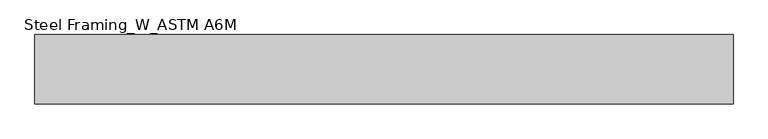
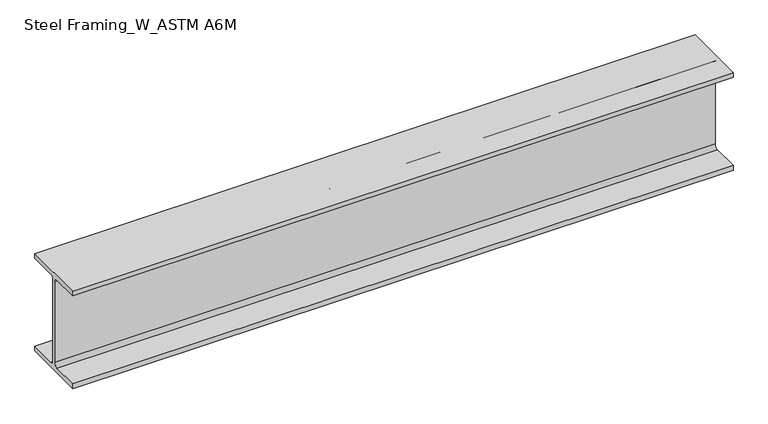
"""IFC4 building model written with IfcOpenShell, lengths in millimetres: beam geometry, Steel Framing_W_ASTM A6M : H_SB_AR_S02_W200x31.3_B6."""

import ifcopenshell
import ifcopenshell.guid

model = None  # the IFC model being written
_history = None  # IfcOwnerHistory: only IFC2X3 demands one
_inside = {}  # id of a spatial element -> (the spatial element, [elements in it])
_under = {}  # id of a project, library or spatial element -> (it, [spatial elements below it])
_declared = {}  # id of a project -> (the project, [libraries it declares])
_typed = {}  # id of a type object -> (the type object, [elements of that type])
_made_of = {}  # id of a material, layer set ... -> (it, [elements and type objects made of it])


def new_model(schema):
    """Start an empty IFC model of exactly this schema.

    Asked for "IFC4X3", IfcOpenShell would pick the latest addendum, in which some entities
    have other attributes; the version numbers below select the first issue.
    IFC2X3 requires an IfcOwnerHistory on every rooted entity: one is made here for all.
    """
    global model, _history
    if schema == "IFC4X3":
        model = ifcopenshell.file(schema_version=(4, 3, 0, 0))
    else:
        model = ifcopenshell.file(schema=schema)
    _inside.clear()
    _under.clear()
    _declared.clear()
    _typed.clear()
    _made_of.clear()
    _history = None
    if model.schema == "IFC2X3":
        org = make("IfcOrganization", Name="unknown")
        user = make(
            "IfcPersonAndOrganization",
            ThePerson=make("IfcPerson", FamilyName="unknown"),
            TheOrganization=org,
        )
        app = make(
            "IfcApplication",
            ApplicationDeveloper=org,
            Version="unknown",
            ApplicationFullName="unknown",
            ApplicationIdentifier="unknown",
        )
        _history = make(
            "IfcOwnerHistory",
            OwningUser=user,
            OwningApplication=app,
            ChangeAction="ADDED",
            CreationDate=0,
        )
    return model


def make(cls, **values):
    """One entity of the class cls with the attributes given. An attribute that is None is left unset."""
    return model.create_entity(
        cls, **{name: value for name, value in values.items() if value is not None}
    )


def rooted(cls, **values):
    """An entity with a GlobalId (a new one), such as an element, a storey or a relation."""
    return make(cls, GlobalId=ifcopenshell.guid.new(), OwnerHistory=_history, **values)


def si_unit(unit_type, name, prefix=None):
    """IfcSIUnit, for example si_unit("LENGTHUNIT", "METRE", prefix="MILLI")."""
    return make("IfcSIUnit", UnitType=unit_type, Prefix=prefix, Name=name)


def assignment(units):
    """IfcUnitAssignment: the units of a project."""
    return None if units is None else make("IfcUnitAssignment", Units=units)


def point(xyz):
    """IfcCartesianPoint."""
    return None if xyz is None else make("IfcCartesianPoint", Coordinates=xyz)


def direction(xyz):
    """IfcDirection."""
    return None if xyz is None else make("IfcDirection", DirectionRatios=xyz)


def frame(location, z_axis=None, x_axis=None):
    """IfcAxis2Placement3D, a coordinate frame: its origin and axes. An axis left out is left unset."""
    return make(
        "IfcAxis2Placement3D",
        Location=point(location),
        Axis=direction(z_axis),
        RefDirection=direction(x_axis),
    )


def frame_2d(location, x_axis=None):
    """IfcAxis2Placement2D, a coordinate frame in the plane: its origin and x axis."""
    return make(
        "IfcAxis2Placement2D", Location=point(location), RefDirection=direction(x_axis)
    )


def origin():
    """The frame at (0, 0, 0) with its axes left unset."""
    return frame((0.0, 0.0, 0.0))


def place(relative_to, where):
    """IfcLocalPlacement: puts the frame where relative to a parent placement (None: the world)."""
    return make(
        "IfcLocalPlacement", PlacementRelTo=relative_to, RelativePlacement=where
    )


def context(
    kind, dimensions, precision=None, world=None, true_north=None, identifier=None
):
    """IfcGeometricRepresentationContext, for example the 3D "Model" context."""
    return make(
        "IfcGeometricRepresentationContext",
        ContextIdentifier=identifier,
        ContextType=kind,
        CoordinateSpaceDimension=dimensions,
        Precision=precision,
        WorldCoordinateSystem=world,
        TrueNorth=true_north,
    )


def project(units=None, contexts=None):
    """IfcProject with its units and contexts."""
    return rooted(
        "IfcProject",
        Name="project",
        RepresentationContexts=contexts,
        UnitsInContext=assignment(units),
    )


def spatial(cls, under=None, at=None, **own):
    """A site, building, storey or space (cls), placed at a placement, below another one or the project."""
    s = rooted(cls, ObjectPlacement=at, **own)
    if under is not None:
        _under.setdefault(under.id(), (under, []))[1].append(s)
    return s


def polyline(points):
    """IfcPolyline through the points."""
    return make("IfcPolyline", Points=[point(p) for p in points])


def circle_curve(where, radius):
    """IfcCircle in the frame where."""
    return make("IfcCircle", Position=where, Radius=radius)


def trimmed(basis, trim1, trim2, sense, master):
    """IfcTrimmedCurve: the piece of a basis curve between two trims."""
    return make(
        "IfcTrimmedCurve",
        BasisCurve=basis,
        Trim1=trim1,
        Trim2=trim2,
        SenseAgreement=sense,
        MasterRepresentation=master,
    )


def segment(curve, same_sense, transition):
    """IfcCompositeCurveSegment."""
    return make(
        "IfcCompositeCurveSegment",
        Transition=transition,
        SameSense=same_sense,
        ParentCurve=curve,
    )


def composite_curve(segments, self_intersect=None):
    """IfcCompositeCurve: segments joined end to end."""
    return make("IfcCompositeCurve", Segments=segments, SelfIntersect=self_intersect)


def outline(outer, holes=None, kind="AREA"):
    """IfcArbitraryClosedProfileDef: a profile drawn as a closed curve; with holes, ...WithVoids."""
    if holes is None:
        return make("IfcArbitraryClosedProfileDef", ProfileType=kind, OuterCurve=outer)
    return make(
        "IfcArbitraryProfileDefWithVoids",
        ProfileType=kind,
        OuterCurve=outer,
        InnerCurves=holes,
    )


def extrude(swept, where, along, depth):
    """IfcExtrudedAreaSolid: the profile swept, set in the frame where, extruded along a direction by depth."""
    return make(
        "IfcExtrudedAreaSolid",
        SweptArea=swept,
        Position=where,
        ExtrudedDirection=direction(along),
        Depth=depth,
    )


def shape(context_of_items, identifier, shape_type, items):
    """IfcShapeRepresentation: the items that make up one representation, for example the "Body"."""
    return make(
        "IfcShapeRepresentation",
        ContextOfItems=context_of_items,
        RepresentationIdentifier=identifier,
        RepresentationType=shape_type,
        Items=items,
    )


def source(mapping_origin, context_of_items, identifier, shape_type, items):
    """IfcRepresentationMap: a shape defined once, which mapped items show again and again."""
    return make(
        "IfcRepresentationMap",
        MappingOrigin=mapping_origin,
        MappedRepresentation=shape(context_of_items, identifier, shape_type, items),
    )


def transform(
    local_origin,
    x_axis=None,
    y_axis=None,
    z_axis=None,
    scale=None,
    scale2=None,
    scale3=None,
    uniform=True,
):
    """IfcCartesianTransformationOperator3D, or its non-uniform kind. x_axis, y_axis, z_axis: its Axis1, 2, 3."""
    if uniform:
        return make(
            "IfcCartesianTransformationOperator3D",
            Axis1=direction(x_axis),
            Axis2=direction(y_axis),
            LocalOrigin=point(local_origin),
            Scale=scale,
            Axis3=direction(z_axis),
        )
    return make(
        "IfcCartesianTransformationOperator3DnonUniform",
        Axis1=direction(x_axis),
        Axis2=direction(y_axis),
        LocalOrigin=point(local_origin),
        Scale=scale,
        Axis3=direction(z_axis),
        Scale2=scale2,
        Scale3=scale3,
    )


def mapped(mapping_source, mapping_target):
    """IfcMappedItem: shows the shape of a source again, moved by a transform."""
    return make(
        "IfcMappedItem", MappingSource=mapping_source, MappingTarget=mapping_target
    )


def made_of(thing, what):
    """Note that an element or type object is made of a material, layer set ...; save() writes the relation."""
    if what is not None:
        _made_of.setdefault(what.id(), (what, []))[1].append(thing)
    return thing


def element(
    cls,
    number,
    at=None,
    inside=None,
    cuts=None,
    type_object=None,
    material=None,
    context=None,
    identifier="Body",
    shape_type=None,
    held_by="IfcProductDefinitionShape",
    body=None,
    shapes=None,
    **own,
):
    """One element of the class cls, such as IfcWall. Its Tag is "e" and its number.

    at: its placement. inside: the storey or other place that contains it. cuts: it is an
    opening in that element (IfcRelVoidsElement). A single representation is given by context,
    identifier, shape_type and body (its items); several are given by shapes. held_by: the class
    of the entity that holds the representations. save() writes the other relations.
    """
    e = rooted(cls, Tag="e%d" % number, ObjectPlacement=at, **own)
    if body is not None:
        shapes = [shape(context, identifier, shape_type, body)]
    if shapes is not None:
        e.Representation = make(held_by, Representations=shapes)
    if inside is not None:
        _inside.setdefault(inside.id(), (inside, []))[1].append(e)
    if cuts is not None:
        rooted(
            "IfcRelVoidsElement", RelatingBuildingElement=cuts, RelatedOpeningElement=e
        )
    if type_object is not None:
        _typed.setdefault(type_object.id(), (type_object, []))[1].append(e)
    return made_of(e, material)


def aggregate(whole, parts):
    """IfcRelAggregates: a whole, such as a stair, and the parts it consists of."""
    return rooted("IfcRelAggregates", RelatingObject=whole, RelatedObjects=parts)


def save(model, path):
    """Write the relations noted so far, then the file.

    IfcRelAggregates (storeys below a building ...), IfcRelContainedInSpatialStructure (elements
    in a storey), IfcRelDefinesByType, IfcRelAssociatesMaterial and IfcRelDeclares: one each for
    every whole, place, type object, material and project.
    """
    for whole, parts in _under.values():
        aggregate(whole, parts)
    for where, things in _inside.values():
        rooted(
            "IfcRelContainedInSpatialStructure",
            RelatedElements=things,
            RelatingStructure=where,
        )
    for kind, things in _typed.values():
        rooted("IfcRelDefinesByType", RelatedObjects=things, RelatingType=kind)
    for what, things in _made_of.values():
        rooted("IfcRelAssociatesMaterial", RelatedObjects=things, RelatingMaterial=what)
    for by, libraries in _declared.values():
        rooted("IfcRelDeclares", RelatingContext=by, RelatedDefinitions=libraries)
    model.write(path)


def steel_framing_w_astm_a6m_deedff07(model_context):
    return source(origin(), model_context, "Body", "SweptSolid", [
        extrude(outline(composite_curve([segment(polyline([(67.0, -94.8), (67.0, -105.0), (-67.0, -105.0), (-67.0, -94.8), (-10.775, -94.8)]), True, "CONTINUOUS"), segment(trimmed(circle_curve(frame_2d((-10.775, -87.2)), 7.6), [point((-10.775, -94.8))], [point((-3.175, -87.2))], True, "CARTESIAN"), True, "CONTINUOUS"), segment(polyline([(-3.175, -87.2), (-3.175, 87.2)]), True, "CONTINUOUS"), segment(trimmed(circle_curve(frame_2d((-10.775, 87.2)), 7.6), [point((-3.175, 87.2))], [point((-10.775, 94.8))], True, "CARTESIAN"), True, "CONTINUOUS"), segment(polyline([(-10.775, 94.8), (-67.0, 94.8), (-67.0, 105.0), (67.0, 105.0), (67.0, 94.8), (10.775, 94.8)]), True, "CONTINUOUS"), segment(trimmed(circle_curve(frame_2d((10.775, 87.2)), 7.6), [point((10.775, 94.8))], [point((3.175, 87.2))], True, "CARTESIAN"), True, "CONTINUOUS"), segment(polyline([(3.175, 87.2), (3.175, -87.2)]), True, "CONTINUOUS"), segment(trimmed(circle_curve(frame_2d((10.775, -87.2)), 7.6), [point((3.175, -87.2))], [point((10.775, -94.8))], True, "CARTESIAN"), True, "CONTINUOUS"), segment(polyline([(10.775, -94.8), (67.0, -94.8)]), True, "CONTINUOUS")], self_intersect=False)), frame((-625.5, 0.0, 0.0), z_axis=(1.0, 0.0, 0.0), x_axis=(0.0, 1.0, 0.0)), (0.0, 0.0, 1.0), 1345.8),
    ])


if __name__ == "__main__":
    model = new_model("IFC4")
    model_context = context("Model", 3, world=origin())
    ifc_project = project(units=[si_unit("LENGTHUNIT", "METRE", prefix="MILLI")], contexts=[model_context])
    site = spatial("IfcSite", under=ifc_project)
    building = spatial("IfcBuilding", under=site)
    placement = place(None, origin())
    steel_framing_w_astm_a6m_shape = steel_framing_w_astm_a6m_deedff07(model_context)
    element("IfcBeam", 1, ObjectType="Steel Framing_W_ASTM A6M : H_SB_AR_S02_W200x31.3_B6", at=placement, inside=building, context=model_context, shape_type="MappedRepresentation", body=[
        mapped(steel_framing_w_astm_a6m_shape, transform((0.0, 0.0, 0.0), x_axis=(1.0, 0.0, 0.0), y_axis=(0.0, 1.0, 0.0), z_axis=(0.0, 0.0, 1.0))),
    ])
    save(model, "model.ifc")

# Revit data of these elements
# Type "Steel Framing_W_ASTM A6M : H_SB_AR_S02_W200x31.3_B6"
#   Type Mark = "B6"
#   Section Name Key = "W8x21"
#   Width = 13.4 cm
#   Web Thickness = 0.635 cm
#   Web Fillet = 0.76 cm
#   Warping Constant = 40800.0 cm⁶
#   Torsional Moment of Inertia = 11.70 cm⁴
#   Section Area = 39.7 cm²
#   Plastic Modulus weak axis = 93.2 cm³
#   Plastic Modulus strong axis = 334.0 cm³
#   Perimeter = 0.93 m²/m
#   Nominal Weight = 31.30 kgf/m
#   Moment of Inertia weak axis = 407.00 cm⁴
#   Moment of Inertia strong axis = 3130.00 cm⁴
#   Height = 21.0 cm
#   Flange Thickness = 1.02 cm
#   Elastic Modulus weak axis = 60.8 cm³
#   Elastic Modulus strong axis = 298.0 cm³
#   Centroid Vertical = 10.5 cm
#   Centroid Horizontal = 6.7 cm
#   Length [instance default] = 1500 mm
#   Structural Material [instance default] = Steel, 45-345
#   Bolt Spacing = 0
#   Assembly Code = ""
# Element 1 (IfcBeam, "Steel Framing_W_ASTM A6M : H_SB_AR_S02_W200x31.3_B6")
#   Materials on its faces: "Steel, 45-345"
# Materials
#   "Steel, 45-345": class "Metal", colour RGB 189 187 185, transparency 0, Description = "Steel 345 MPa", Cost = 0
